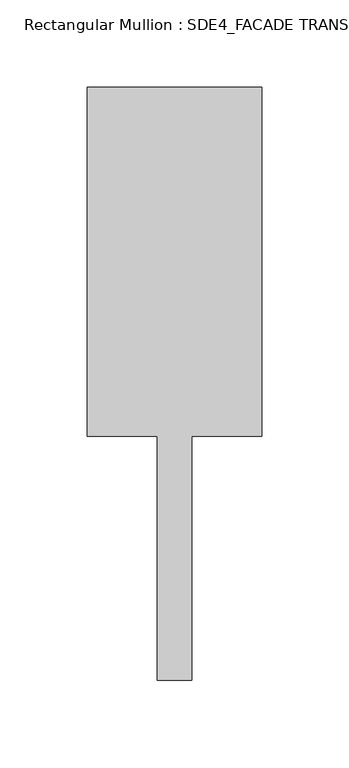
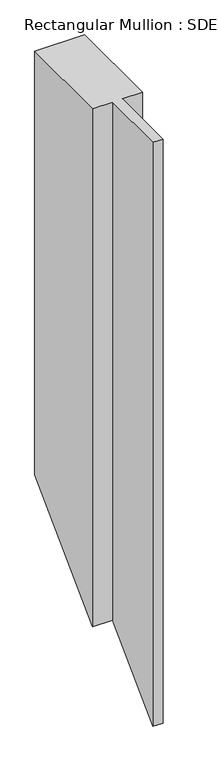
"""IFC4 building model written with IfcOpenShell, lengths in millimetres: member geometry, Rectangular Mullion : SDE4_FACADE TRANSOM TYPE 1."""

import ifcopenshell
import ifcopenshell.guid

model = None  # the IFC model being written
_history = None  # IfcOwnerHistory: only IFC2X3 demands one
_inside = {}  # id of a spatial element -> (the spatial element, [elements in it])
_under = {}  # id of a project, library or spatial element -> (it, [spatial elements below it])
_declared = {}  # id of a project -> (the project, [libraries it declares])
_typed = {}  # id of a type object -> (the type object, [elements of that type])
_made_of = {}  # id of a material, layer set ... -> (it, [elements and type objects made of it])


def new_model(schema):
    """Start an empty IFC model of exactly this schema.

    Asked for "IFC4X3", IfcOpenShell would pick the latest addendum, in which some entities
    have other attributes; the version numbers below select the first issue.
    IFC2X3 requires an IfcOwnerHistory on every rooted entity: one is made here for all.
    """
    global model, _history
    if schema == "IFC4X3":
        model = ifcopenshell.file(schema_version=(4, 3, 0, 0))
    else:
        model = ifcopenshell.file(schema=schema)
    _inside.clear()
    _under.clear()
    _declared.clear()
    _typed.clear()
    _made_of.clear()
    _history = None
    if model.schema == "IFC2X3":
        org = make("IfcOrganization", Name="unknown")
        user = make(
            "IfcPersonAndOrganization",
            ThePerson=make("IfcPerson", FamilyName="unknown"),
            TheOrganization=org,
        )
        app = make(
            "IfcApplication",
            ApplicationDeveloper=org,
            Version="unknown",
            ApplicationFullName="unknown",
            ApplicationIdentifier="unknown",
        )
        _history = make(
            "IfcOwnerHistory",
            OwningUser=user,
            OwningApplication=app,
            ChangeAction="ADDED",
            CreationDate=0,
        )
    return model


def make(cls, **values):
    """One entity of the class cls with the attributes given. An attribute that is None is left unset."""
    return model.create_entity(
        cls, **{name: value for name, value in values.items() if value is not None}
    )


def rooted(cls, **values):
    """An entity with a GlobalId (a new one), such as an element, a storey or a relation."""
    return make(cls, GlobalId=ifcopenshell.guid.new(), OwnerHistory=_history, **values)


def si_unit(unit_type, name, prefix=None):
    """IfcSIUnit, for example si_unit("LENGTHUNIT", "METRE", prefix="MILLI")."""
    return make("IfcSIUnit", UnitType=unit_type, Prefix=prefix, Name=name)


def assignment(units):
    """IfcUnitAssignment: the units of a project."""
    return None if units is None else make("IfcUnitAssignment", Units=units)


def point(xyz):
    """IfcCartesianPoint."""
    return None if xyz is None else make("IfcCartesianPoint", Coordinates=xyz)


def direction(xyz):
    """IfcDirection."""
    return None if xyz is None else make("IfcDirection", DirectionRatios=xyz)


def frame(location, z_axis=None, x_axis=None):
    """IfcAxis2Placement3D, a coordinate frame: its origin and axes. An axis left out is left unset."""
    return make(
        "IfcAxis2Placement3D",
        Location=point(location),
        Axis=direction(z_axis),
        RefDirection=direction(x_axis),
    )


def origin():
    """The frame at (0, 0, 0) with its axes left unset."""
    return frame((0.0, 0.0, 0.0))


def place(relative_to, where):
    """IfcLocalPlacement: puts the frame where relative to a parent placement (None: the world)."""
    return make(
        "IfcLocalPlacement", PlacementRelTo=relative_to, RelativePlacement=where
    )


def context(
    kind, dimensions, precision=None, world=None, true_north=None, identifier=None
):
    """IfcGeometricRepresentationContext, for example the 3D "Model" context."""
    return make(
        "IfcGeometricRepresentationContext",
        ContextIdentifier=identifier,
        ContextType=kind,
        CoordinateSpaceDimension=dimensions,
        Precision=precision,
        WorldCoordinateSystem=world,
        TrueNorth=true_north,
    )


def project(units=None, contexts=None):
    """IfcProject with its units and contexts."""
    return rooted(
        "IfcProject",
        Name="project",
        RepresentationContexts=contexts,
        UnitsInContext=assignment(units),
    )


def spatial(cls, under=None, at=None, **own):
    """A site, building, storey or space (cls), placed at a placement, below another one or the project."""
    s = rooted(cls, ObjectPlacement=at, **own)
    if under is not None:
        _under.setdefault(under.id(), (under, []))[1].append(s)
    return s


def faces_of(points, faces, orient=None, outer=None):
    """IfcFace entities. A face is a list of loops; a loop is a list of indices into points, from 0.

    orient and outer hold one flag for each loop. By default every Orientation is true, the
    first loop of a face is its IfcFaceOuterBound and the others are IfcFaceBound.
    """
    made = []
    for i, loops in enumerate(faces):
        bounds = []
        for j, loop in enumerate(loops):
            is_outer = j == 0 if outer is None else outer[i][j]
            bounds.append(
                make(
                    "IfcFaceOuterBound" if is_outer else "IfcFaceBound",
                    Bound=make("IfcPolyLoop", Polygon=[points[k] for k in loop]),
                    Orientation=True if orient is None else orient[i][j],
                )
            )
        made.append(make("IfcFace", Bounds=bounds))
    return made


def faceted_brep(points, faces, orient=None, outer=None, voids=None):
    """IfcFacetedBrep: a solid bounded by flat faces; with voids (closed shells), ...WithVoids."""
    shared = [point(p) for p in points]
    hull = make("IfcClosedShell", CfsFaces=faces_of(shared, faces, orient, outer))
    if voids is None:
        return make("IfcFacetedBrep", Outer=hull)
    return make(
        "IfcFacetedBrepWithVoids",
        Outer=hull,
        Voids=[
            make(cls, CfsFaces=faces_of(shared, fs, o, b)) for cls, fs, o, b in voids
        ],
    )


def shape(context_of_items, identifier, shape_type, items):
    """IfcShapeRepresentation: the items that make up one representation, for example the "Body"."""
    return make(
        "IfcShapeRepresentation",
        ContextOfItems=context_of_items,
        RepresentationIdentifier=identifier,
        RepresentationType=shape_type,
        Items=items,
    )


def source(mapping_origin, context_of_items, identifier, shape_type, items):
    """IfcRepresentationMap: a shape defined once, which mapped items show again and again."""
    return make(
        "IfcRepresentationMap",
        MappingOrigin=mapping_origin,
        MappedRepresentation=shape(context_of_items, identifier, shape_type, items),
    )


def transform(
    local_origin,
    x_axis=None,
    y_axis=None,
    z_axis=None,
    scale=None,
    scale2=None,
    scale3=None,
    uniform=True,
):
    """IfcCartesianTransformationOperator3D, or its non-uniform kind. x_axis, y_axis, z_axis: its Axis1, 2, 3."""
    if uniform:
        return make(
            "IfcCartesianTransformationOperator3D",
            Axis1=direction(x_axis),
            Axis2=direction(y_axis),
            LocalOrigin=point(local_origin),
            Scale=scale,
            Axis3=direction(z_axis),
        )
    return make(
        "IfcCartesianTransformationOperator3DnonUniform",
        Axis1=direction(x_axis),
        Axis2=direction(y_axis),
        LocalOrigin=point(local_origin),
        Scale=scale,
        Axis3=direction(z_axis),
        Scale2=scale2,
        Scale3=scale3,
    )


def mapped(mapping_source, mapping_target):
    """IfcMappedItem: shows the shape of a source again, moved by a transform."""
    return make(
        "IfcMappedItem", MappingSource=mapping_source, MappingTarget=mapping_target
    )


def made_of(thing, what):
    """Note that an element or type object is made of a material, layer set ...; save() writes the relation."""
    if what is not None:
        _made_of.setdefault(what.id(), (what, []))[1].append(thing)
    return thing


def element(
    cls,
    number,
    at=None,
    inside=None,
    cuts=None,
    type_object=None,
    material=None,
    context=None,
    identifier="Body",
    shape_type=None,
    held_by="IfcProductDefinitionShape",
    body=None,
    shapes=None,
    **own,
):
    """One element of the class cls, such as IfcWall. Its Tag is "e" and its number.

    at: its placement. inside: the storey or other place that contains it. cuts: it is an
    opening in that element (IfcRelVoidsElement). A single representation is given by context,
    identifier, shape_type and body (its items); several are given by shapes. held_by: the class
    of the entity that holds the representations. save() writes the other relations.
    """
    e = rooted(cls, Tag="e%d" % number, ObjectPlacement=at, **own)
    if body is not None:
        shapes = [shape(context, identifier, shape_type, body)]
    if shapes is not None:
        e.Representation = make(held_by, Representations=shapes)
    if inside is not None:
        _inside.setdefault(inside.id(), (inside, []))[1].append(e)
    if cuts is not None:
        rooted(
            "IfcRelVoidsElement", RelatingBuildingElement=cuts, RelatedOpeningElement=e
        )
    if type_object is not None:
        _typed.setdefault(type_object.id(), (type_object, []))[1].append(e)
    return made_of(e, material)


def aggregate(whole, parts):
    """IfcRelAggregates: a whole, such as a stair, and the parts it consists of."""
    return rooted("IfcRelAggregates", RelatingObject=whole, RelatedObjects=parts)


def save(model, path):
    """Write the relations noted so far, then the file.

    IfcRelAggregates (storeys below a building ...), IfcRelContainedInSpatialStructure (elements
    in a storey), IfcRelDefinesByType, IfcRelAssociatesMaterial and IfcRelDeclares: one each for
    every whole, place, type object, material and project.
    """
    for whole, parts in _under.values():
        aggregate(whole, parts)
    for where, things in _inside.values():
        rooted(
            "IfcRelContainedInSpatialStructure",
            RelatedElements=things,
            RelatingStructure=where,
        )
    for kind, things in _typed.values():
        rooted("IfcRelDefinesByType", RelatedObjects=things, RelatingType=kind)
    for what, things in _made_of.values():
        rooted("IfcRelAssociatesMaterial", RelatedObjects=things, RelatingMaterial=what)
    for by, libraries in _declared.values():
        rooted("IfcRelDeclares", RelatingContext=by, RelatedDefinitions=libraries)
    model.write(path)


def rectangular_mullion_sde4_facade_transom_type_1_1d4a49a0(model_context):
    return source(origin(), model_context, "Body", "Brep", [
        faceted_brep([(50.0, 132.5, 0.0), (-50.0, 132.5, 0.0), (-50.0, -67.5, 0.0), (-10.0, -67.5, 0.0), (-10.0, -207.5, 0.0), (10.0, -207.5, 0.0), (10.0, -67.5, 0.0), (50.0, -67.5, 0.0), (50.0, 132.5, -893.75), (-50.0, 132.5, -893.75), (-50.0, -67.5, -1093.75), (-10.0, -67.5, -1093.75), (-10.0, -207.5, -1233.75), (10.0, -207.5, -1233.75), (10.0, -67.5, -1093.75), (50.0, -67.5, -1093.75)], [[[0, 1, 2, 3, 4, 5, 6, 7]], [[1, 0, 8, 9]], [[2, 1, 9, 10]], [[3, 2, 10, 11]], [[4, 3, 11, 12]], [[5, 4, 12, 13]], [[6, 5, 13, 14]], [[7, 6, 14, 15]], [[0, 7, 15, 8]], [[8, 15, 14, 13, 12, 11, 10, 9]]]),
    ])


if __name__ == "__main__":
    model = new_model("IFC4")
    model_context = context("Model", 3, world=origin())
    ifc_project = project(units=[si_unit("LENGTHUNIT", "METRE", prefix="MILLI")], contexts=[model_context])
    site = spatial("IfcSite", under=ifc_project)
    building = spatial("IfcBuilding", under=site)
    placement = place(None, origin())
    rectangular_mullion_sde4_facade_transom_type_1_shape = rectangular_mullion_sde4_facade_transom_type_1_1d4a49a0(model_context)
    element("IfcMember", 1, ObjectType="Rectangular Mullion : SDE4_FACADE TRANSOM TYPE 1", at=placement, inside=building, context=model_context, shape_type="MappedRepresentation", body=[
        mapped(rectangular_mullion_sde4_facade_transom_type_1_shape, transform((0.0, 0.0, 0.0), x_axis=(1.0, 0.0, 0.0), y_axis=(0.0, 1.0, 0.0), z_axis=(0.0, 0.0, 1.0))),
    ])
    save(model, "model.ifc")

# Revit data of these elements
# Type "Rectangular Mullion : SDE4_FACADE TRANSOM TYPE 1"
#   built-in parameter 1007322 = 1.11549 (stored number, unit not read)
#   built-in parameter 1007321 = 0.164042 (stored number, unit not read)
#   built-in parameter 1007320 = 0.164042 (stored number, unit not read)
